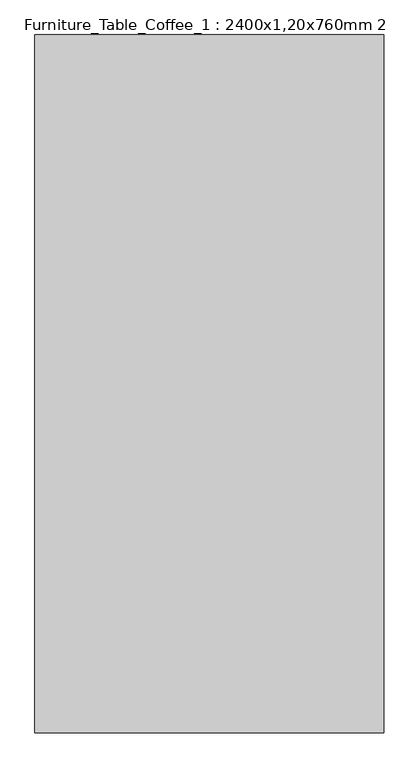
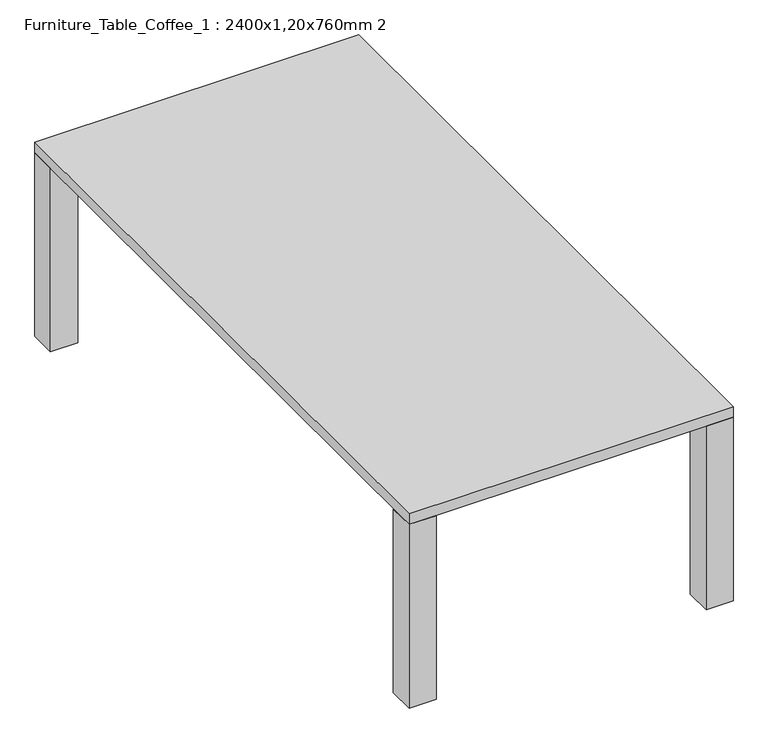
"""IFC4 building model written with IfcOpenShell, lengths in millimetres: furniture geometry, Furniture_Table_Coffee_1 : 2400x1,20x760mm 2."""

from ifc_helpers import new_model, si_unit, frame, origin, origin_with_axes, place, context, project, spatial, polyline, outline, extrude, source, transform, mapped, element, save


def furniture_table_coffee_1_2400x1_20x760mm_2_8aca478b(model_context):
    return source(origin(), model_context, "Body", "SweptSolid", [
        extrude(outline(polyline([(-849.0981188, 839.3758368), (-849.0981188, 739.3758368), (-949.0981188, 739.3758368), (-949.0981188, 839.3758368), (-849.0981188, 839.3758368)])), origin_with_axes(), (0.0, 0.0, 1.0), 718.6),
        extrude(outline(polyline([(250.9018812, 839.3758368), (250.9018812, 739.3758368), (150.9018812, 739.3758368), (150.9018812, 839.3758368), (250.9018812, 839.3758368)])), origin_with_axes(), (0.0, 0.0, 1.0), 718.6),
        extrude(outline(polyline([(250.9018812, -1460.6241632), (250.9018812, -1560.6241632), (150.9018812, -1560.6241632), (150.9018812, -1460.6241632), (250.9018812, -1460.6241632)])), origin_with_axes(), (0.0, 0.0, 1.0), 718.6),
        extrude(outline(polyline([(-949.0981188, -1460.6241632), (-849.0981188, -1460.6241632), (-849.0981188, -1560.6241632), (-949.0981188, -1560.6241632), (-949.0981188, -1460.6241632)])), origin_with_axes(), (0.0, 0.0, 1.0), 718.6),
        extrude(outline(polyline([(250.9018812, 839.3758368), (250.9018812, -1560.6241632), (-949.0981188, -1560.6241632), (-949.0981188, 839.3758368), (250.9018812, 839.3758368)])), frame((0.0, 0.0, 718.6), z_axis=(0.0, 0.0, 1.0), x_axis=(1.0, 0.0, 0.0)), (0.0, 0.0, 1.0), 41.4),
    ])


if __name__ == "__main__":
    model = new_model("IFC4")
    model_context = context("Model", 3, world=origin())
    ifc_project = project(units=[si_unit("LENGTHUNIT", "METRE", prefix="MILLI")], contexts=[model_context])
    site = spatial("IfcSite", under=ifc_project)
    building = spatial("IfcBuilding", under=site)
    placement = place(None, origin())
    furniture_table_coffee_1_2400x1_20x760mm_2_shape = furniture_table_coffee_1_2400x1_20x760mm_2_8aca478b(model_context)
    element("IfcFurniture", 1, ObjectType="Furniture_Table_Coffee_1 : 2400x1,20x760mm 2", at=placement, inside=building, context=model_context, shape_type="MappedRepresentation", body=[
        mapped(furniture_table_coffee_1_2400x1_20x760mm_2_shape, transform((0.0, 0.0, 0.0), x_axis=(1.0, 0.0, 0.0), y_axis=(0.0, 1.0, 0.0), z_axis=(0.0, 0.0, 1.0))),
    ])
    save(model, "model.ifc")

# Revit data of these elements
# Type "Furniture_Table_Coffee_1 : 2400x1,20x760mm 2"
#   Type IfcGUID = "34sfOaXm13ZR3byzHHycup"
#   Keynote = "N"
#   Model = "FVGB23"
#   Manufacturer = "Revit"
#   Description = "Coffee table"
#   Assembly Code = "E2020200"
#   Cost = 99
#   Length = 2.4 m
#   Width = 1.2 m
#   Leg Width = 0.1 m
#   Height = 0.76 m
#   Material = Plastic - Grey
#   Type Comments = ""
#   Default Elevation = 0
#   Cost = 0
# Element 1 (IfcFurniture, "Furniture_Table_Coffee_1 : 2400x1,20x760mm 2")
#   Materials on its faces: "Plastic - Grey"
# Materials
#   "Plastic - Grey": class "Plastic", colour RGB 162 162 162, transparency 0
